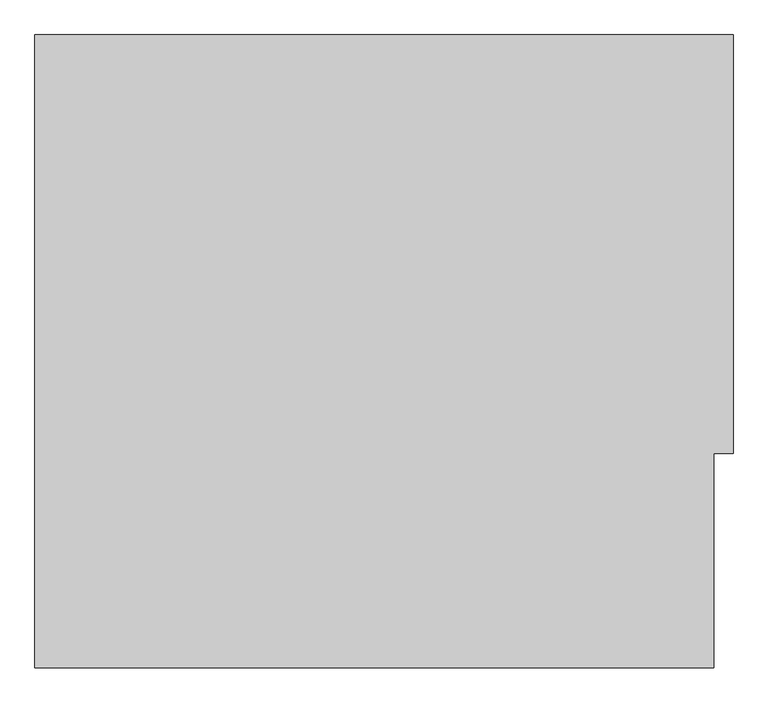
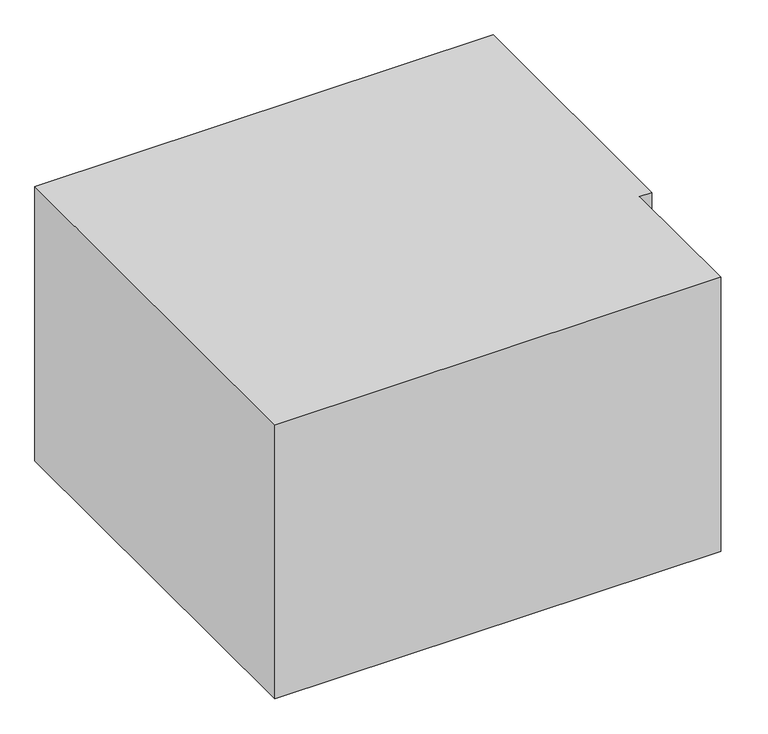
"""IFC4 building model written with IfcOpenShell, lengths in millimetres: proxy geometry, 0_3d."""

from ifc_helpers import new_model, si_unit, origin, origin_with_axes, place, context, project, spatial, polyline, outline, extrude, source, transform, mapped, element, save


def generic_models_9102e70f(model_context):
    return source(origin(), model_context, "Body", "SweptSolid", [
        extrude(outline(polyline([(4425.0, 1395.9795824), (4425.0, 0.0), (0.0, 0.0), (0.0, 4125.9795824), (4550.0, 4125.9795824), (4550.0, 1395.9795824), (4425.0, 1395.9795824)])), origin_with_axes(), (0.0, 0.0, 1.0), 2880.0),
    ])


if __name__ == "__main__":
    model = new_model("IFC4")
    model_context = context("Model", 3, world=origin())
    ifc_project = project(units=[si_unit("LENGTHUNIT", "METRE", prefix="MILLI")], contexts=[model_context])
    site = spatial("IfcSite", under=ifc_project)
    building = spatial("IfcBuilding", under=site)
    placement = place(None, origin())
    generic_models_shape = generic_models_9102e70f(model_context)
    element("IfcBuildingElementProxy", 1, Name="0_3d", ObjectType="0_3d", at=placement, inside=building, context=model_context, shape_type="MappedRepresentation", body=[
        mapped(generic_models_shape, transform((0.0, 0.0, 0.0), x_axis=(1.0, 0.0, 0.0), y_axis=(0.0, 1.0, 0.0), z_axis=(0.0, 0.0, 1.0))),
    ])
    save(model, "model.ifc")

# Revit data of these elements
# Element 1 (IfcBuildingElementProxy, "0_3d")
#   Materials on its faces: "*1"
# Materials
#   "*1": class "Unassigned", colour RGB 175 175 175, transparency 0
